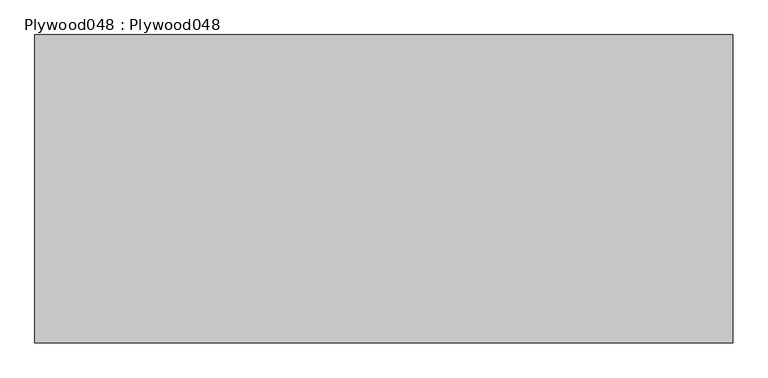
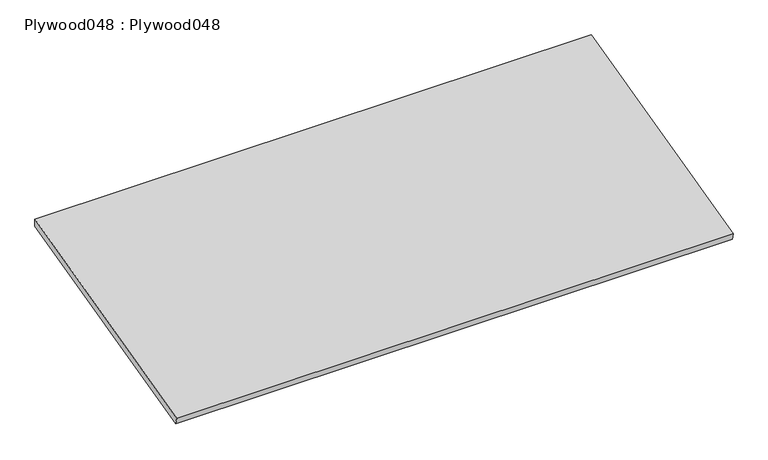
"""IFC4 building model written with IfcOpenShell, lengths in millimetres: proxy geometry, Plywood048 : Plywood048."""

from ifc_helpers import new_model, si_unit, frame, origin, place, context, project, spatial, polyline, outline, extrude, source, transform, mapped, element, save


def plywood048_plywood048_3e493ecb(model_context):
    return source(origin(), model_context, "Body", "SweptSolid", [
        extrude(outline(polyline([(-4222.1357939, 42658.3302851), (-4228.2961988, 42682.9719046), (-3344.6566162, 42903.8818003), (-3344.6566162, 42877.7000796), (-4222.1357939, 42658.3302851)])), frame((12383.0178845, 0.0, 0.0), z_axis=(1.0, 0.0, 0.0), x_axis=(0.0, 1.0, 0.0)), (0.0, 0.0, 1.0), 2000.0),
    ])


if __name__ == "__main__":
    model = new_model("IFC4")
    model_context = context("Model", 3, world=origin())
    ifc_project = project(units=[si_unit("LENGTHUNIT", "METRE", prefix="MILLI")], contexts=[model_context])
    site = spatial("IfcSite", under=ifc_project)
    building = spatial("IfcBuilding", under=site)
    placement = place(None, origin())
    plywood048_plywood048_shape = plywood048_plywood048_3e493ecb(model_context)
    element("IfcBuildingElementProxy", 1, Name="Plywood048 : Plywood048", ObjectType="Plywood048 : Plywood048", at=placement, inside=building, context=model_context, shape_type="MappedRepresentation", body=[
        mapped(plywood048_plywood048_shape, transform((0.0, 0.0, 0.0), x_axis=(1.0, 0.0, 0.0), y_axis=(0.0, 1.0, 0.0), z_axis=(0.0, 0.0, 1.0))),
    ])
    save(model, "model.ifc")

# Revit data of these elements
# Type "Plywood048 : Plywood048"
#   NameOverride = "Plywood048"
# Element 1 (IfcBuildingElementProxy, "Plywood048 : Plywood048")
#   Materials on its faces: "WHITE OAK CEILING OVER VAPOR BARRIER"
# Materials
#   "WHITE OAK CEILING OVER VAPOR BARRIER": class "Unassigned", colour RGB 227 188 136, transparency 0, Cost = 0
